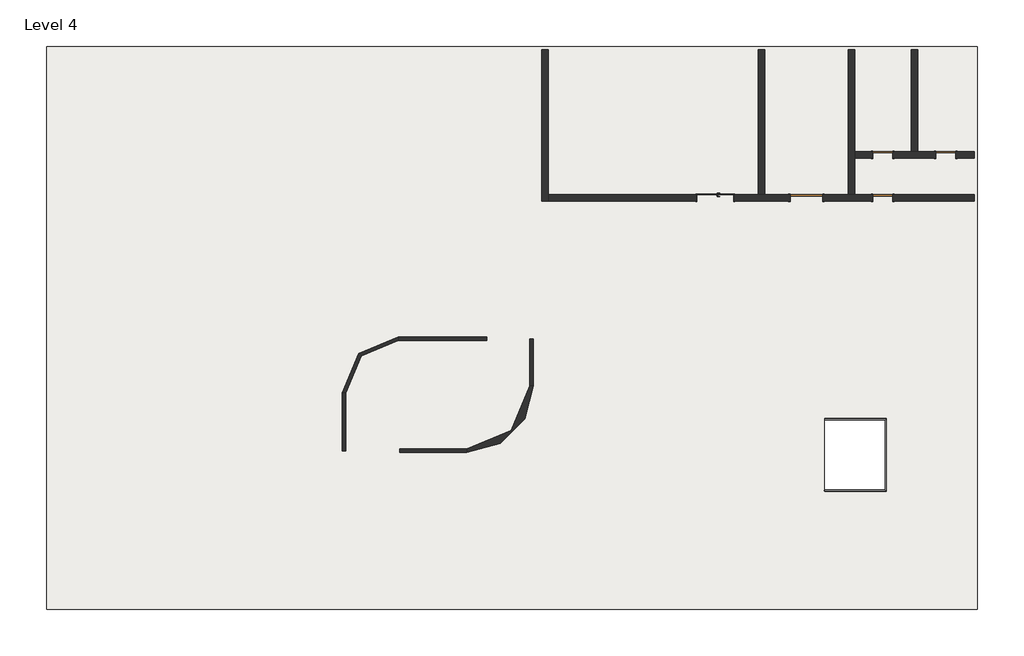
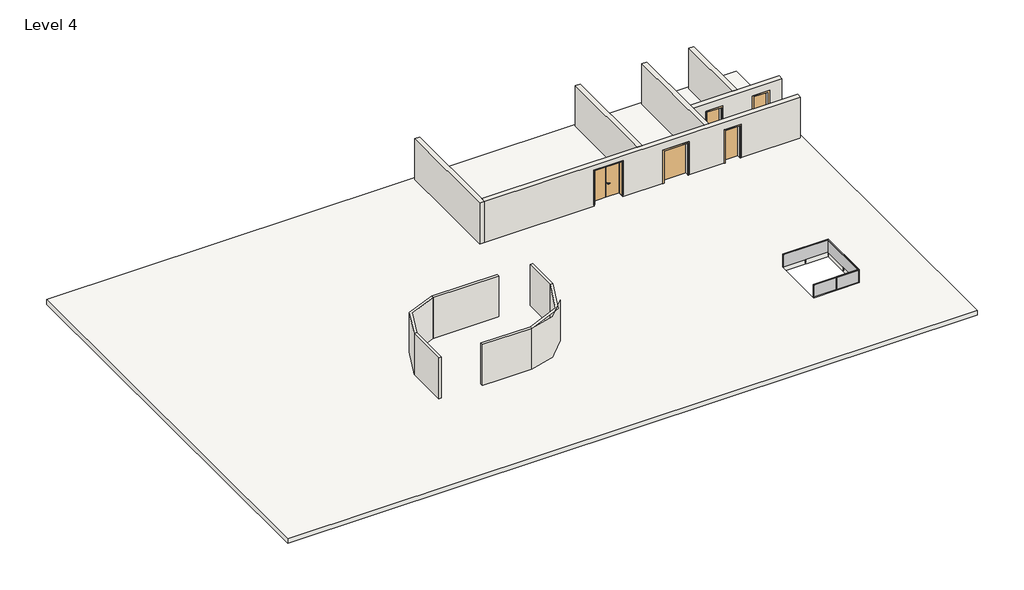
# One storey: 12 walls, 5 doors, 1 railing, 1 slab.
"""IFC4 building model written with IfcOpenShell, lengths in millimetres."""

import ifcopenshell
import ifcopenshell.guid

model = None  # the IFC model being written
_history = None  # IfcOwnerHistory: only IFC2X3 demands one
_inside = {}  # id of a spatial element -> (the spatial element, [elements in it])
_under = {}  # id of a project, library or spatial element -> (it, [spatial elements below it])
_declared = {}  # id of a project -> (the project, [libraries it declares])
_typed = {}  # id of a type object -> (the type object, [elements of that type])
_made_of = {}  # id of a material, layer set ... -> (it, [elements and type objects made of it])


def new_model(schema):
    """Start an empty IFC model of exactly this schema.

    Asked for "IFC4X3", IfcOpenShell would pick the latest addendum, in which some entities
    have other attributes; the version numbers below select the first issue.
    IFC2X3 requires an IfcOwnerHistory on every rooted entity: one is made here for all.
    """
    global model, _history
    if schema == "IFC4X3":
        model = ifcopenshell.file(schema_version=(4, 3, 0, 0))
    else:
        model = ifcopenshell.file(schema=schema)
    _inside.clear()
    _under.clear()
    _declared.clear()
    _typed.clear()
    _made_of.clear()
    _history = None
    if model.schema == "IFC2X3":
        org = make("IfcOrganization", Name="unknown")
        user = make(
            "IfcPersonAndOrganization",
            ThePerson=make("IfcPerson", FamilyName="unknown"),
            TheOrganization=org,
        )
        app = make(
            "IfcApplication",
            ApplicationDeveloper=org,
            Version="unknown",
            ApplicationFullName="unknown",
            ApplicationIdentifier="unknown",
        )
        _history = make(
            "IfcOwnerHistory",
            OwningUser=user,
            OwningApplication=app,
            ChangeAction="ADDED",
            CreationDate=0,
        )
    return model


def make(cls, **values):
    """One entity of the class cls with the attributes given. An attribute that is None is left unset."""
    return model.create_entity(
        cls, **{name: value for name, value in values.items() if value is not None}
    )


def rooted(cls, **values):
    """An entity with a GlobalId (a new one), such as an element, a storey or a relation."""
    return make(cls, GlobalId=ifcopenshell.guid.new(), OwnerHistory=_history, **values)


def si_unit(unit_type, name, prefix=None):
    """IfcSIUnit, for example si_unit("LENGTHUNIT", "METRE", prefix="MILLI")."""
    return make("IfcSIUnit", UnitType=unit_type, Prefix=prefix, Name=name)


def assignment(units):
    """IfcUnitAssignment: the units of a project."""
    return None if units is None else make("IfcUnitAssignment", Units=units)


def point(xyz):
    """IfcCartesianPoint."""
    return None if xyz is None else make("IfcCartesianPoint", Coordinates=xyz)


def direction(xyz):
    """IfcDirection."""
    return None if xyz is None else make("IfcDirection", DirectionRatios=xyz)


def frame(location, z_axis=None, x_axis=None):
    """IfcAxis2Placement3D, a coordinate frame: its origin and axes. An axis left out is left unset."""
    return make(
        "IfcAxis2Placement3D",
        Location=point(location),
        Axis=direction(z_axis),
        RefDirection=direction(x_axis),
    )


def frame_2d(location, x_axis=None):
    """IfcAxis2Placement2D, a coordinate frame in the plane: its origin and x axis."""
    return make(
        "IfcAxis2Placement2D", Location=point(location), RefDirection=direction(x_axis)
    )


def origin():
    """The frame at (0, 0, 0) with its axes left unset."""
    return frame((0.0, 0.0, 0.0))


def origin_with_axes():
    """The frame at (0, 0, 0) with the z axis (0, 0, 1) and the x axis (1, 0, 0) written out."""
    return frame((0.0, 0.0, 0.0), z_axis=(0.0, 0.0, 1.0), x_axis=(1.0, 0.0, 0.0))


def place(relative_to, where):
    """IfcLocalPlacement: puts the frame where relative to a parent placement (None: the world)."""
    return make(
        "IfcLocalPlacement", PlacementRelTo=relative_to, RelativePlacement=where
    )


def context(
    kind, dimensions, precision=None, world=None, true_north=None, identifier=None
):
    """IfcGeometricRepresentationContext, for example the 3D "Model" context."""
    return make(
        "IfcGeometricRepresentationContext",
        ContextIdentifier=identifier,
        ContextType=kind,
        CoordinateSpaceDimension=dimensions,
        Precision=precision,
        WorldCoordinateSystem=world,
        TrueNorth=true_north,
    )


def project(units=None, contexts=None):
    """IfcProject with its units and contexts."""
    return rooted(
        "IfcProject",
        Name="project",
        RepresentationContexts=contexts,
        UnitsInContext=assignment(units),
    )


def spatial(cls, under=None, at=None, **own):
    """A site, building, storey or space (cls), placed at a placement, below another one or the project."""
    s = rooted(cls, ObjectPlacement=at, **own)
    if under is not None:
        _under.setdefault(under.id(), (under, []))[1].append(s)
    return s


def polyline(points):
    """IfcPolyline through the points."""
    return make("IfcPolyline", Points=[point(p) for p in points])


def circle_curve(where, radius):
    """IfcCircle in the frame where."""
    return make("IfcCircle", Position=where, Radius=radius)


def ellipse_curve(where, semi_axis1, semi_axis2):
    """IfcEllipse in the frame where."""
    return make(
        "IfcEllipse", Position=where, SemiAxis1=semi_axis1, SemiAxis2=semi_axis2
    )


def trimmed(basis, trim1, trim2, sense, master):
    """IfcTrimmedCurve: the piece of a basis curve between two trims."""
    return make(
        "IfcTrimmedCurve",
        BasisCurve=basis,
        Trim1=trim1,
        Trim2=trim2,
        SenseAgreement=sense,
        MasterRepresentation=master,
    )


def segment(curve, same_sense, transition):
    """IfcCompositeCurveSegment."""
    return make(
        "IfcCompositeCurveSegment",
        Transition=transition,
        SameSense=same_sense,
        ParentCurve=curve,
    )


def composite_curve(segments, self_intersect=None):
    """IfcCompositeCurve: segments joined end to end."""
    return make("IfcCompositeCurve", Segments=segments, SelfIntersect=self_intersect)


def outline(outer, holes=None, kind="AREA"):
    """IfcArbitraryClosedProfileDef: a profile drawn as a closed curve; with holes, ...WithVoids."""
    if holes is None:
        return make("IfcArbitraryClosedProfileDef", ProfileType=kind, OuterCurve=outer)
    return make(
        "IfcArbitraryProfileDefWithVoids",
        ProfileType=kind,
        OuterCurve=outer,
        InnerCurves=holes,
    )


def extrude(swept, where, along, depth):
    """IfcExtrudedAreaSolid: the profile swept, set in the frame where, extruded along a direction by depth."""
    return make(
        "IfcExtrudedAreaSolid",
        SweptArea=swept,
        Position=where,
        ExtrudedDirection=direction(along),
        Depth=depth,
    )


def faces_of(points, faces, orient=None, outer=None):
    """IfcFace entities. A face is a list of loops; a loop is a list of indices into points, from 0.

    orient and outer hold one flag for each loop. By default every Orientation is true, the
    first loop of a face is its IfcFaceOuterBound and the others are IfcFaceBound.
    """
    made = []
    for i, loops in enumerate(faces):
        bounds = []
        for j, loop in enumerate(loops):
            is_outer = j == 0 if outer is None else outer[i][j]
            bounds.append(
                make(
                    "IfcFaceOuterBound" if is_outer else "IfcFaceBound",
                    Bound=make("IfcPolyLoop", Polygon=[points[k] for k in loop]),
                    Orientation=True if orient is None else orient[i][j],
                )
            )
        made.append(make("IfcFace", Bounds=bounds))
    return made


def faceted_brep(points, faces, orient=None, outer=None, voids=None):
    """IfcFacetedBrep: a solid bounded by flat faces; with voids (closed shells), ...WithVoids."""
    shared = [point(p) for p in points]
    hull = make("IfcClosedShell", CfsFaces=faces_of(shared, faces, orient, outer))
    if voids is None:
        return make("IfcFacetedBrep", Outer=hull)
    return make(
        "IfcFacetedBrepWithVoids",
        Outer=hull,
        Voids=[
            make(cls, CfsFaces=faces_of(shared, fs, o, b)) for cls, fs, o, b in voids
        ],
    )


def shape(context_of_items, identifier, shape_type, items):
    """IfcShapeRepresentation: the items that make up one representation, for example the "Body"."""
    return make(
        "IfcShapeRepresentation",
        ContextOfItems=context_of_items,
        RepresentationIdentifier=identifier,
        RepresentationType=shape_type,
        Items=items,
    )


def source(mapping_origin, context_of_items, identifier, shape_type, items):
    """IfcRepresentationMap: a shape defined once, which mapped items show again and again."""
    return make(
        "IfcRepresentationMap",
        MappingOrigin=mapping_origin,
        MappedRepresentation=shape(context_of_items, identifier, shape_type, items),
    )


def transform(
    local_origin,
    x_axis=None,
    y_axis=None,
    z_axis=None,
    scale=None,
    scale2=None,
    scale3=None,
    uniform=True,
):
    """IfcCartesianTransformationOperator3D, or its non-uniform kind. x_axis, y_axis, z_axis: its Axis1, 2, 3."""
    if uniform:
        return make(
            "IfcCartesianTransformationOperator3D",
            Axis1=direction(x_axis),
            Axis2=direction(y_axis),
            LocalOrigin=point(local_origin),
            Scale=scale,
            Axis3=direction(z_axis),
        )
    return make(
        "IfcCartesianTransformationOperator3DnonUniform",
        Axis1=direction(x_axis),
        Axis2=direction(y_axis),
        LocalOrigin=point(local_origin),
        Scale=scale,
        Axis3=direction(z_axis),
        Scale2=scale2,
        Scale3=scale3,
    )


def mapped(mapping_source, mapping_target):
    """IfcMappedItem: shows the shape of a source again, moved by a transform."""
    return make(
        "IfcMappedItem", MappingSource=mapping_source, MappingTarget=mapping_target
    )


def made_of(thing, what):
    """Note that an element or type object is made of a material, layer set ...; save() writes the relation."""
    if what is not None:
        _made_of.setdefault(what.id(), (what, []))[1].append(thing)
    return thing


def element(
    cls,
    number,
    at=None,
    inside=None,
    cuts=None,
    type_object=None,
    material=None,
    context=None,
    identifier="Body",
    shape_type=None,
    held_by="IfcProductDefinitionShape",
    body=None,
    shapes=None,
    **own,
):
    """One element of the class cls, such as IfcWall. Its Tag is "e" and its number.

    at: its placement. inside: the storey or other place that contains it. cuts: it is an
    opening in that element (IfcRelVoidsElement). A single representation is given by context,
    identifier, shape_type and body (its items); several are given by shapes. held_by: the class
    of the entity that holds the representations. save() writes the other relations.
    """
    e = rooted(cls, Tag="e%d" % number, ObjectPlacement=at, **own)
    if body is not None:
        shapes = [shape(context, identifier, shape_type, body)]
    if shapes is not None:
        e.Representation = make(held_by, Representations=shapes)
    if inside is not None:
        _inside.setdefault(inside.id(), (inside, []))[1].append(e)
    if cuts is not None:
        rooted(
            "IfcRelVoidsElement", RelatingBuildingElement=cuts, RelatedOpeningElement=e
        )
    if type_object is not None:
        _typed.setdefault(type_object.id(), (type_object, []))[1].append(e)
    return made_of(e, material)


def aggregate(whole, parts):
    """IfcRelAggregates: a whole, such as a stair, and the parts it consists of."""
    return rooted("IfcRelAggregates", RelatingObject=whole, RelatedObjects=parts)


def save(model, path):
    """Write the relations noted so far, then the file.

    IfcRelAggregates (storeys below a building ...), IfcRelContainedInSpatialStructure (elements
    in a storey), IfcRelDefinesByType, IfcRelAssociatesMaterial and IfcRelDeclares: one each for
    every whole, place, type object, material and project.
    """
    for whole, parts in _under.values():
        aggregate(whole, parts)
    for where, things in _inside.values():
        rooted(
            "IfcRelContainedInSpatialStructure",
            RelatedElements=things,
            RelatingStructure=where,
        )
    for kind, things in _typed.values():
        rooted("IfcRelDefinesByType", RelatedObjects=things, RelatingType=kind)
    for what, things in _made_of.values():
        rooted("IfcRelAssociatesMaterial", RelatedObjects=things, RelatingMaterial=what)
    for by, libraries in _declared.values():
        rooted("IfcRelDeclares", RelatingContext=by, RelatedDefinitions=libraries)
    model.write(path)


def plane_surface(at):
    """IfcPlane: the flat surface through the origin of the frame at, square to its z axis."""
    return make("IfcPlane", Position=at)


def cylinder_surface(at, radius):
    """IfcCylindricalSurface: all points at the distance radius from the z axis of the frame at."""
    return make("IfcCylindricalSurface", Position=at, Radius=radius)


def advanced_brep(points, edges, surfaces, faces):
    """IfcAdvancedBrep: a solid bounded by faces that lie on surfaces and meet in shared edges.

    An edge is (start, end): straight between two places in points (the first is 0);
    or (start, end, curve); or (start, end, curve, False) where it runs against its curve.
    A face is (place in surfaces, loops), or (place, loops, False) where it looks against
    its surface's normal. A loop lists edges by number (the first is 1), with a minus sign
    where the edge is run from its end to its start. The first loop is the outer one.
    """
    corners = [point(p) for p in points]
    vertices = [make("IfcVertexPoint", VertexGeometry=c) for c in corners]
    made = []
    for start, end, *more in edges:
        made.append(
            make(
                "IfcEdgeCurve",
                EdgeStart=vertices[start],
                EdgeEnd=vertices[end],
                EdgeGeometry=more[0] if more else make("IfcPolyline", Points=[corners[start], corners[end]]),
                SameSense=more[1] if len(more) > 1 else True,
            )
        )
    hull = []
    for where, loops, *sense in faces:
        bounds = []
        for j, loop in enumerate(loops):
            ring = [make("IfcOrientedEdge", EdgeElement=made[abs(k) - 1], Orientation=k > 0) for k in loop]
            bounds.append(
                make(
                    "IfcFaceOuterBound" if j == 0 else "IfcFaceBound",
                    Bound=make("IfcEdgeLoop", EdgeList=ring),
                    Orientation=True,
                )
            )
        hull.append(make("IfcAdvancedFace", Bounds=bounds, FaceSurface=surfaces[where], SameSense=sense[0] if sense else True))
    return make("IfcAdvancedBrep", Outer=make("IfcClosedShell", CfsFaces=hull))


def door_double_flush_variable_door_double_flush_variable_ac6c3b87(model_context):
    return source(origin(), model_context, "Body", "SolidModel", [
        advanced_brep(
        [(90.0, 139.4346141, 1000.0), (110.0, 139.4346141, 1000.0), (90.0, 69.4346141, 1000.0), (110.0, 89.4346141, 1000.0), (220.0, 69.4346141, 1000.0), (220.0, 89.4346141, 1000.0)],
        [
            (0, 1, circle_curve(frame((100.0, 139.4346141, 1000.0), z_axis=(0.0, 1.0, 0.0), x_axis=(1.0, 0.0, 0.0)), 10.0)),
            (1, 0, circle_curve(frame((100.0, 139.4346141, 1000.0), z_axis=(0.0, 1.0, 0.0), x_axis=(1.0, 0.0, 0.0)), 10.0)),
            (0, 2),
            (2, 3, ellipse_curve(frame((100.0, 79.4346141, 1000.0), z_axis=(-0.7071067811865385, 0.7071067811865565, 0.0), x_axis=(0.7071067811865563, 0.7071067811865386, 0.0)), 14.1421356, 10.0)),
            (3, 1),
            (3, 2, ellipse_curve(frame((100.0, 79.4346141, 1000.0), z_axis=(-0.7071067811865385, 0.7071067811865565, 0.0), x_axis=(0.7071067811865563, 0.7071067811865386, 0.0)), 14.1421356, 10.0)),
            (4, 5, circle_curve(frame((220.0, 79.4346141, 1000.0), z_axis=(1.0, 0.0, 0.0), x_axis=(0.0, 1.0, 0.0)), 10.0)),
            (5, 4, circle_curve(frame((220.0, 79.4346141, 1000.0), z_axis=(1.0, 0.0, 0.0), x_axis=(0.0, 1.0, 0.0)), 10.0)),
            (2, 4),
            (5, 3),
        ],
        [
            plane_surface(frame((100.0, 139.4346141, -287.7526403), z_axis=(0.0, 1.0, 0.0), x_axis=(0.0, 0.0, 1.0))),
            cylinder_surface(frame((100.0, 139.4346141, 1000.0), z_axis=(0.0, 1.0, 0.0), x_axis=(1.0, 0.0, 0.0)), 10.0),
            plane_surface(frame((220.0, 79.4346141, -287.7526403), z_axis=(1.0, 0.0, 0.0), x_axis=(0.0, 0.0, 1.0))),
            cylinder_surface(frame((100.0, 79.4346141, 1000.0), z_axis=(-1.0, 0.0, 0.0), x_axis=(0.0, 1.0, 0.0)), 10.0),
        ],
        [
            (0, [[1, 2]]),
            (1, [[-1, 3, 4, 5]]),
            (1, [[-2, -5, 6, -3]]),
            (2, [[7, 8]]),
            (3, [[-4, 9, -8, 10]]),
            (3, [[-6, -10, -7, -9]]),
        ],
    ),
        advanced_brep(
        [(110.0, 199.4346141, 1000.0), (90.0, 199.4346141, 1000.0), (110.0, 229.4346141, 1000.0), (90.0, 249.4346141, 1000.0), (220.0, 229.4346141, 1000.0), (220.0, 249.4346141, 1000.0)],
        [
            (0, 1, circle_curve(frame((100.0, 199.4346141, 1000.0), z_axis=(0.0, -1.0, 0.0), x_axis=(-1.0, 0.0, 0.0)), 10.0)),
            (1, 0, circle_curve(frame((100.0, 199.4346141, 1000.0), z_axis=(0.0, -1.0, 0.0), x_axis=(-1.0, 0.0, 0.0)), 10.0)),
            (0, 2),
            (2, 3, ellipse_curve(frame((100.0, 239.4346141, 1000.0), z_axis=(-0.7071067811865475, -0.7071067811865475, 0.0), x_axis=(0.7071067811865474, -0.7071067811865476, 0.0)), 14.1421356, 10.0)),
            (3, 1),
            (3, 2, ellipse_curve(frame((100.0, 239.4346141, 1000.0), z_axis=(-0.7071067811865475, -0.7071067811865475, 0.0), x_axis=(0.7071067811865474, -0.7071067811865476, 0.0)), 14.1421356, 10.0)),
            (4, 5, circle_curve(frame((220.0, 239.4346141, 1000.0), z_axis=(1.0, 0.0, 0.0), x_axis=(0.0, 1.0, 0.0)), 10.0)),
            (5, 4, circle_curve(frame((220.0, 239.4346141, 1000.0), z_axis=(1.0, 0.0, 0.0), x_axis=(0.0, 1.0, 0.0)), 10.0)),
            (2, 4),
            (5, 3),
        ],
        [
            plane_surface(frame((100.0, 199.4346141, -287.7526403), z_axis=(0.0, -1.0, 0.0), x_axis=(0.0, 0.0, 1.0))),
            cylinder_surface(frame((100.0, 199.4346141, 1000.0), z_axis=(0.0, -1.0, 0.0), x_axis=(-1.0, 0.0, 0.0)), 10.0),
            plane_surface(frame((220.0, 239.4346141, -287.7526403), z_axis=(1.0, 0.0, 0.0), x_axis=(0.0, 0.0, 1.0))),
            cylinder_surface(frame((100.0, 239.4346141, 1000.0), z_axis=(-1.0, 0.0, 0.0), x_axis=(0.0, 1.0, 0.0)), 10.0),
        ],
        [
            (0, [[1, 2]]),
            (1, [[-1, 3, 4, 5]]),
            (1, [[-2, -5, 6, -3]]),
            (2, [[7, 8]]),
            (3, [[-4, 9, -8, 10]]),
            (3, [[-6, -10, -7, -9]]),
        ],
    ),
        extrude(outline(composite_curve([segment(trimmed(circle_curve(frame_2d((1000.0, 100.0)), 20.0), [point((1000.0, 80.0))], [point((1000.0, 120.0))], False, "CARTESIAN"), True, "CONTINUOUS"), segment(trimmed(circle_curve(frame_2d((1000.0, 100.0)), 20.0), [point((1000.0, 120.0))], [point((1000.0, 80.0))], False, "CARTESIAN"), True, "CONTINUOUS")], self_intersect=False)), frame((0.0, 129.4346141, 0.0), z_axis=(0.0, 1.0, 0.0), x_axis=(0.0, 0.0, 1.0)), (0.0, 0.0, 1.0), 10.0),
        extrude(outline(composite_curve([segment(trimmed(circle_curve(frame_2d((1000.0, 100.0)), 20.0), [point((1000.0, 80.0))], [point((1000.0, 120.0))], False, "CARTESIAN"), True, "CONTINUOUS"), segment(trimmed(circle_curve(frame_2d((1000.0, 100.0)), 20.0), [point((1000.0, 120.0))], [point((1000.0, 80.0))], False, "CARTESIAN"), True, "CONTINUOUS")], self_intersect=False)), frame((0.0, 189.4346141, 0.0), z_axis=(0.0, 1.0, 0.0), x_axis=(0.0, 0.0, 1.0)), (0.0, 0.0, 1.0), 10.0),
        extrude(outline(polyline([(0.0, 164.4346141), (-871.25, 164.4346141), (-871.25, 189.4346141), (0.0, 189.4346141), (0.0, 164.4346141)])), frame((0.0, 0.0, 100.0), z_axis=(0.0, 0.0, 1.0), x_axis=(1.0, 0.0, 0.0)), (0.0, 0.0, 1.0), 2250.0),
        extrude(outline(polyline([(871.25, 164.4346141), (0.0, 164.4346141), (0.0, 189.4346141), (871.25, 189.4346141), (871.25, 164.4346141)])), frame((0.0, 0.0, 100.0), z_axis=(0.0, 0.0, 1.0), x_axis=(1.0, 0.0, 0.0)), (0.0, 0.0, 1.0), 2250.0),
        faceted_brep([(905.75, -150.5653859, 100.0), (856.25, -150.5653859, 100.0), (856.25, 164.4346141, 100.0), (871.25, 164.4346141, 100.0), (871.25, 189.4346141, 100.0), (905.75, 189.4346141, 100.0), (905.75, 164.4346141, 100.0), (900.75, 164.4346141, 100.0), (900.75, 184.4346141, 100.0), (876.25, 184.4346141, 100.0), (876.25, 159.4346141, 100.0), (861.25, 159.4346141, 100.0), (861.25, -145.5653859, 100.0), (900.75, -145.5653859, 100.0), (900.75, -135.5653859, 100.0), (905.75, -135.5653859, 100.0), (905.75, -150.5653859, 2384.5), (-905.75, -150.5653859, 2384.5), (-905.75, -150.5653859, 100.0), (-856.25, -150.5653859, 100.0), (-856.25, -150.5653859, 2335.0), (856.25, -150.5653859, 2335.0), (856.25, 164.4346141, 2335.0), (-856.25, 164.4346141, 2335.0), (-856.25, 164.4346141, 100.0), (-871.25, 164.4346141, 100.0), (-871.25, 164.4346141, 2350.0), (871.25, 164.4346141, 2350.0), (871.25, 189.4346141, 2350.0), (-871.25, 189.4346141, 2350.0), (-871.25, 189.4346141, 100.0), (-905.75, 189.4346141, 100.0), (-905.75, 189.4346141, 2384.5), (905.75, 189.4346141, 2384.5), (905.75, 164.4346141, 2384.5), (-905.75, 164.4346141, 2384.5), (-905.75, 164.4346141, 100.0), (-900.75, 164.4346141, 100.0), (-900.75, 164.4346141, 2379.5), (900.75, 164.4346141, 2379.5), (900.75, 184.4346141, 2379.5), (-900.75, 184.4346141, 2379.5), (-900.75, 184.4346141, 100.0), (-876.25, 184.4346141, 100.0), (-876.25, 184.4346141, 2355.0), (876.25, 184.4346141, 2355.0), (876.25, 159.4346141, 2355.0), (-876.25, 159.4346141, 2355.0), (-876.25, 159.4346141, 100.0), (-861.25, 159.4346141, 100.0), (-861.25, 159.4346141, 2340.0), (861.25, 159.4346141, 2340.0), (861.25, -145.5653859, 2340.0), (-861.25, -145.5653859, 2340.0), (-861.25, -145.5653859, 100.0), (-900.75, -145.5653859, 100.0), (-900.75, -145.5653859, 2379.5), (900.75, -145.5653859, 2379.5), (900.75, -135.5653859, 2379.5), (-900.75, -135.5653859, 2379.5), (-900.75, -135.5653859, 100.0), (-905.75, -135.5653859, 100.0), (-905.75, -135.5653859, 2384.5), (905.75, -135.5653859, 2384.5)], [[[0, 1, 2, 3, 4, 5, 6, 7, 8, 9, 10, 11, 12, 13, 14, 15]], [[1, 0, 16, 17, 18, 19, 20, 21]], [[2, 1, 21, 22]], [[3, 2, 22, 23, 24, 25, 26, 27]], [[4, 3, 27, 28]], [[5, 4, 28, 29, 30, 31, 32, 33]], [[6, 5, 33, 34]], [[7, 6, 34, 35, 36, 37, 38, 39]], [[8, 7, 39, 40]], [[9, 8, 40, 41, 42, 43, 44, 45]], [[10, 9, 45, 46]], [[11, 10, 46, 47, 48, 49, 50, 51]], [[12, 11, 51, 52]], [[13, 12, 52, 53, 54, 55, 56, 57]], [[14, 13, 57, 58]], [[15, 14, 58, 59, 60, 61, 62, 63]], [[0, 15, 63, 16]], [[17, 62, 61, 18]], [[18, 61, 60, 55, 54, 49, 48, 43, 42, 37, 36, 31, 30, 25, 24, 19]], [[23, 20, 19, 24]], [[29, 26, 25, 30]], [[35, 32, 31, 36]], [[41, 38, 37, 42]], [[47, 44, 43, 48]], [[53, 50, 49, 54]], [[59, 56, 55, 60]], [[22, 21, 20, 23]], [[28, 27, 26, 29]], [[34, 33, 32, 35]], [[40, 39, 38, 41]], [[46, 45, 44, 47]], [[52, 51, 50, 53]], [[58, 57, 56, 59]], [[16, 63, 62, 17]]]),
    ])


def m_single_flush_0915_x_2134mm_1c84716f(model_context):
    return source(origin(), model_context, "Body", "SweptSolid", [
        extrude(outline(polyline([(2210.0, -533.5), (0.0, -533.5), (0.0, -457.5), (2134.0, -457.5), (2134.0, 457.5), (0.0, 457.5), (0.0, 533.5), (2210.0, 533.5), (2210.0, -533.5)])), frame((0.0, -175.0, 0.0), z_axis=(0.0, 1.0, 0.0), x_axis=(0.0, 0.0, 1.0)), (0.0, 0.0, 1.0), 25.0),
        extrude(outline(polyline([(2210.0, 533.5), (2210.0, -533.5), (0.0, -533.5), (0.0, -457.5), (2134.0, -457.5), (2134.0, 457.5), (0.0, 457.5), (0.0, 533.5), (2210.0, 533.5)])), frame((0.0, 150.0, 0.0), z_axis=(0.0, 1.0, 0.0), x_axis=(0.0, 0.0, 1.0)), (0.0, 0.0, 1.0), 25.0),
        extrude(outline(polyline([(457.5, -99.0), (457.5, -150.0), (-457.5, -150.0), (-457.5, -99.0), (457.5, -99.0)])), origin_with_axes(), (0.0, 0.0, 1.0), 2134.0),
    ])


def m_single_flush_1500_x_2134mm_2_edebd810(model_context):
    return source(origin(), model_context, "Body", "SweptSolid", [
        extrude(outline(polyline([(2210.0, -826.0), (0.0, -826.0), (0.0, -750.0), (2134.0, -750.0), (2134.0, 750.0), (0.0, 750.0), (0.0, 826.0), (2210.0, 826.0), (2210.0, -826.0)])), frame((0.0, -175.0, 0.0), z_axis=(0.0, 1.0, 0.0), x_axis=(0.0, 0.0, 1.0)), (0.0, 0.0, 1.0), 25.0),
        extrude(outline(polyline([(2210.0, 826.0), (2210.0, -826.0), (0.0, -826.0), (0.0, -750.0), (2134.0, -750.0), (2134.0, 750.0), (0.0, 750.0), (0.0, 826.0), (2210.0, 826.0)])), frame((0.0, 150.0, 0.0), z_axis=(0.0, 1.0, 0.0), x_axis=(0.0, 0.0, 1.0)), (0.0, 0.0, 1.0), 25.0),
        extrude(outline(polyline([(750.0, -99.0), (750.0, -150.0), (-750.0, -150.0), (-750.0, -99.0), (750.0, -99.0)])), origin_with_axes(), (0.0, 0.0, 1.0), 2134.0),
    ])


def glas_mpk_6e7e974a(model_context):
    return source(origin(), model_context, "Body", "SolidModel", [
        faceted_brep([(29194.1667192, -1196.642277, 9843.2628643), (29194.1667192, -1246.642277, 9843.2628643), (29194.1667192, -1246.642277, 9856.7371357), (29194.1667192, -1196.642277, 9856.7371357), (32034.1667192, -1196.642277, 9843.2628643), (31984.1667192, -1246.642277, 9843.2628643), (31984.1667192, -1246.642277, 9856.7371357), (32034.1667192, -1196.642277, 9856.7371357), (32034.1667192, -4537.3716232, 9843.2628643), (31984.1667192, -4487.3716232, 9843.2628643), (31984.1667192, -4487.3716232, 9856.7371357), (32034.1667192, -4537.3716232, 9856.7371357), (29194.1667192, -4537.3716232, 9843.2628643), (29194.1667192, -4537.3716232, 9856.7371357), (29194.1667192, -4487.3716232, 9856.7371357), (29194.1667192, -4487.3716232, 9843.2628643)], [[[0, 1, 2, 3]], [[1, 0, 4, 5]], [[2, 1, 5, 6]], [[3, 2, 6, 7]], [[0, 3, 7, 4]], [[5, 4, 8, 9]], [[6, 5, 9, 10]], [[7, 6, 10, 11]], [[4, 7, 11, 8]], [[12, 13, 14, 15]], [[9, 8, 12, 15]], [[10, 9, 15, 14]], [[11, 10, 14, 13]], [[8, 11, 13, 12]]]),
        faceted_brep([(29194.1667192, -1236.642277, 9842.8769824), (29194.1667192, -1222.4501531, 9842.8769824), (29194.1667192, -1222.4501531, 9042.8769824), (29194.1667192, -1236.642277, 9042.8769824), (31994.1667192, -1236.642277, 9842.8769824), (32008.3588432, -1222.4501531, 9842.8769824), (32008.3588432, -1222.4501531, 9042.8769824), (31994.1667192, -1236.642277, 9042.8769824), (31994.1667192, -4497.3716232, 9842.8769824), (32008.3588432, -4511.5637472, 9842.8769824), (32008.3588432, -4511.5637472, 9042.8769824), (31994.1667192, -4497.3716232, 9042.8769824), (29194.1667192, -4497.3716232, 9842.8769824), (29194.1667192, -4497.3716232, 9042.8769824), (29194.1667192, -4511.5637472, 9042.8769824), (29194.1667192, -4511.5637472, 9842.8769824)], [[[0, 1, 2, 3]], [[1, 0, 4, 5]], [[2, 1, 5, 6]], [[3, 2, 6, 7]], [[0, 3, 7, 4]], [[5, 4, 8, 9]], [[6, 5, 9, 10]], [[7, 6, 10, 11]], [[4, 7, 11, 8]], [[12, 13, 14, 15]], [[9, 8, 12, 15]], [[10, 9, 15, 14]], [[11, 10, 14, 13]], [[8, 11, 13, 12]]]),
        extrude(outline(polyline([(30625.4167192, -4512.3716232), (30625.4167192, -4537.3716232), (30600.4167192, -4537.3716232), (30600.4167192, -4512.3716232), (30625.4167192, -4512.3716232)])), frame((0.0, 0.0, 8800.0), z_axis=(0.0, 0.0, 1.0), x_axis=(1.0, 0.0, 0.0)), (0.0, 0.0, 1.0), 1043.2628643),
        extrude(outline(polyline([(32009.1667192, -2854.5069501), (32034.1667192, -2854.5069501), (32034.1667192, -2879.5069501), (32009.1667192, -2879.5069501), (32009.1667192, -2854.5069501)])), frame((0.0, 0.0, 8800.0), z_axis=(0.0, 0.0, 1.0), x_axis=(1.0, 0.0, 0.0)), (0.0, 0.0, 1.0), 1043.2628643),
        extrude(outline(polyline([(30600.4167192, -1221.642277), (30600.4167192, -1196.642277), (30625.4167192, -1196.642277), (30625.4167192, -1221.642277), (30600.4167192, -1221.642277)])), frame((0.0, 0.0, 8800.0), z_axis=(0.0, 0.0, 1.0), x_axis=(1.0, 0.0, 0.0)), (0.0, 0.0, 1.0), 1043.2628643),
        extrude(outline(polyline([(32009.1667192, -4522.3716232), (32034.1667192, -4522.3716232), (32034.1667192, -4547.3716232), (32009.1667192, -4547.3716232), (32009.1667192, -4522.3716232)])), frame((0.0, 0.0, 8800.0), z_axis=(0.0, 0.0, 1.0), x_axis=(1.0, 0.0, 0.0)), (0.0, 0.0, 1.0), 1043.2628643),
        extrude(outline(polyline([(32019.1667192, -1221.642277), (32019.1667192, -1196.642277), (32044.1667192, -1196.642277), (32044.1667192, -1221.642277), (32019.1667192, -1221.642277)])), frame((0.0, 0.0, 8800.0), z_axis=(0.0, 0.0, 1.0), x_axis=(1.0, 0.0, 0.0)), (0.0, 0.0, 1.0), 1043.2628643),
        extrude(outline(polyline([(29206.6667192, -4512.3716232), (29206.6667192, -4537.3716232), (29181.6667192, -4537.3716232), (29181.6667192, -4512.3716232), (29206.6667192, -4512.3716232)])), frame((0.0, 0.0, 8800.0), z_axis=(0.0, 0.0, 1.0), x_axis=(1.0, 0.0, 0.0)), (0.0, 0.0, 1.0), 1043.2628643),
        extrude(outline(polyline([(29194.1667192, -1221.642277), (29194.1667192, -1196.642277), (29219.1667192, -1196.642277), (29219.1667192, -1221.642277), (29194.1667192, -1221.642277)])), frame((0.0, 0.0, 8800.0), z_axis=(0.0, 0.0, 1.0), x_axis=(1.0, 0.0, 0.0)), (0.0, 0.0, 1.0), 1043.2628643),
    ])


model = new_model("IFC4")

# Units and contexts
model_context = context("Model", 3, world=origin())
ifc_project = project(units=[si_unit("LENGTHUNIT", "METRE", prefix="MILLI")], contexts=[model_context])

# Site, building, storey
site = spatial("IfcSite", under=ifc_project)
building = spatial("IfcBuilding", under=site)
storey = spatial("IfcBuildingStorey", under=building, Name="Level 4", Elevation=9000.0)

# Doors
placement = place(None, origin())
door_double_flush_variable_door_double_flush_variable_shape = door_double_flush_variable_door_double_flush_variable_ac6c3b87(model_context)
element("IfcDoor", 1, ObjectType="Door Double Flush - Variable : Door Double Flush - Variable", at=placement, inside=storey, context=model_context, shape_type="MappedRepresentation", body=[
    mapped(door_double_flush_variable_door_double_flush_variable_shape, transform((24136.7471367, 8984.3231089, 9000.0), x_axis=(1.0, 0.0, 0.0), y_axis=(0.0, 1.0, 0.0), z_axis=(0.0, 0.0, 1.0))),
])
m_single_flush_0915_x_2134mm_shape = m_single_flush_0915_x_2134mm_1c84716f(model_context)
element("IfcDoor", 2, ObjectType="M_Single-Flush : 0915 x 2134mm", at=placement, inside=storey, context=model_context, shape_type="MappedRepresentation", body=[
    mapped(m_single_flush_0915_x_2134mm_shape, transform((34787.1221367, 10998.757723, 9000.0), x_axis=(-1.0, 0.0, 0.0), y_axis=(0.0, -1.0, 0.0), z_axis=(0.0, 0.0, 1.0))),
])
element("IfcDoor", 3, ObjectType="M_Single-Flush : 0915 x 2134mm", at=placement, inside=storey, context=model_context, shape_type="MappedRepresentation", body=[
    mapped(m_single_flush_0915_x_2134mm_shape, transform((31874.3721367, 10998.757723, 9000.0), x_axis=(-1.0, 0.0, 0.0), y_axis=(0.0, -1.0, 0.0), z_axis=(0.0, 0.0, 1.0))),
])
element("IfcDoor", 4, ObjectType="M_Single-Flush : 0915 x 2134mm", at=placement, inside=storey, context=model_context, shape_type="MappedRepresentation", body=[
    mapped(m_single_flush_0915_x_2134mm_shape, transform((31874.3721367, 8998.757723, 9000.0), x_axis=(-1.0, 0.0, 0.0), y_axis=(0.0, -1.0, 0.0), z_axis=(0.0, 0.0, 1.0))),
])
m_single_flush_1500_x_2134mm_2_shape = m_single_flush_1500_x_2134mm_2_edebd810(model_context)
element("IfcDoor", 5, ObjectType="M_Single-Flush : 1500 x 2134mm 2", at=placement, inside=storey, context=model_context, shape_type="MappedRepresentation", body=[
    mapped(m_single_flush_1500_x_2134mm_2_shape, transform((28342.9971367, 8998.757723, 9000.0), x_axis=(-1.0, 0.0, 0.0), y_axis=(0.0, -1.0, 0.0), z_axis=(0.0, 0.0, 1.0))),
])

# Railing
glas_mpk_shape = glas_mpk_6e7e974a(model_context)
element("IfcRailing", 6, ObjectType="Glas - MPK", at=placement, inside=storey, context=model_context, shape_type="MappedRepresentation", body=[
    mapped(glas_mpk_shape, transform((0.0, 0.0, 0.0), x_axis=(1.0, 0.0, 0.0), y_axis=(0.0, 1.0, 0.0), z_axis=(0.0, 0.0, 1.0))),
])

# Slab
element("IfcSlab", 7, ObjectType="Generic 300mm", at=placement, inside=storey, context=model_context, shape_type="SweptSolid", body=[
    extrude(outline(polyline([(-6732.0028633, 15998.757723), (36243.4971367, 15998.757723), (36243.4971367, -10001.242277), (-6732.0028633, -10001.242277), (-6732.0028633, 15998.757723)]), holes=[polyline([(32044.1667192, -1186.642277), (29194.1667192, -1186.642277), (29194.1667192, -4547.3716232), (32044.1667192, -4547.3716232), (32044.1667192, -1186.642277)])]), frame((0.0, 0.0, 8700.0), z_axis=(0.0, 0.0, 1.0), x_axis=(1.0, 0.0, 0.0)), (0.0, 0.0, 1.0), 300.0),
])

# Walls
element("IfcWall", 8, ObjectType="Generic - 300mm", at=placement, inside=storey, context=model_context, shape_type="Brep", body=[
    faceted_brep([(16117.9971367, 15848.757723, 9000.0), (16117.9971367, 8848.757723, 9000.0), (16117.9971367, 8848.757723, 11700.0), (16117.9971367, 15848.757723, 11700.0), (16417.9971367, 15848.757723, 9000.0), (16417.9971367, 15848.757723, 11700.0), (16417.9971367, 9148.757723, 11700.0), (16417.9971367, 8848.757723, 11700.0), (16417.9971367, 8848.757723, 9000.0), (16417.9971367, 9148.757723, 9000.0)], [[[0, 1, 2, 3]], [[4, 5, 6, 7, 8, 9]], [[1, 0, 4, 9, 8]], [[3, 2, 7, 6, 5]], [[2, 1, 8, 7]], [[0, 3, 5, 4]]]),
])
element("IfcWall", 9, ObjectType="Generic - 300mm", at=placement, inside=storey, context=model_context, shape_type="SweptSolid", body=[
    extrude(outline(polyline([(26117.9971367, 9148.757723), (26117.9971367, 15848.757723), (26417.9971367, 15848.757723), (26417.9971367, 9148.757723), (26117.9971367, 9148.757723)])), frame((0.0, 0.0, 9000.0), z_axis=(0.0, 0.0, 1.0), x_axis=(1.0, 0.0, 0.0)), (0.0, 0.0, 1.0), 2700.0),
])
element("IfcWall", 10, ObjectType="Generic - 300mm", at=placement, inside=storey, context=model_context, shape_type="Brep", body=[
    faceted_brep([(30267.9971367, 15848.757723, 9000.0), (30267.9971367, 9148.757723, 9000.0), (30267.9971367, 9148.757723, 11700.0), (30267.9971367, 15848.757723, 11700.0), (30567.9971367, 15848.757723, 9000.0), (30567.9971367, 15848.757723, 11700.0), (30567.9971367, 11148.757723, 11700.0), (30567.9971367, 10848.757723, 11700.0), (30567.9971367, 9148.757723, 11700.0), (30567.9971367, 9148.757723, 9000.0), (30567.9971367, 10848.757723, 9000.0), (30567.9971367, 11148.757723, 9000.0)], [[[0, 1, 2, 3]], [[4, 5, 6, 7, 8, 9, 10, 11]], [[1, 0, 4, 11, 10, 9]], [[3, 2, 8, 7, 6, 5]], [[2, 1, 9, 8]], [[0, 3, 5, 4]]]),
])
element("IfcWall", 11, ObjectType="Generic - 300mm", at=placement, inside=storey, context=model_context, shape_type="SweptSolid", body=[
    extrude(outline(polyline([(33180.7471367, 11148.757723), (33180.7471367, 15848.757723), (33480.7471367, 15848.757723), (33480.7471367, 11148.757723), (33180.7471367, 11148.757723)])), frame((0.0, 0.0, 9000.0), z_axis=(0.0, 0.0, 1.0), x_axis=(1.0, 0.0, 0.0)), (0.0, 0.0, 1.0), 2700.0),
])
element("IfcWall", 12, ObjectType="Generic - 300mm", at=placement, inside=storey, context=model_context, shape_type="Brep", body=[
    faceted_brep([(16417.9971367, 9148.757723, 11700.0), (26117.9971367, 9148.757723, 11700.0), (26417.9971367, 9148.757723, 11700.0), (30267.9971367, 9148.757723, 11700.0), (30567.9971367, 9148.757723, 11700.0), (36093.4971367, 9148.757723, 11700.0), (36093.4971367, 9148.757723, 9000.0), (32331.8721367, 9148.757723, 9000.0), (32331.8721367, 9148.757723, 11134.0), (31416.8721367, 9148.757723, 11134.0), (31416.8721367, 9148.757723, 9000.0), (30567.9971367, 9148.757723, 9000.0), (30267.9971367, 9148.757723, 9000.0), (29092.9971367, 9148.757723, 9000.0), (29092.9971367, 9148.757723, 11134.0), (27592.9971367, 9148.757723, 11134.0), (27592.9971367, 9148.757723, 9000.0), (26417.9971367, 9148.757723, 9000.0), (26117.9971367, 9148.757723, 9000.0), (25017.9971367, 9148.757723, 9000.0), (25017.9971367, 9148.757723, 11360.0), (23255.4971367, 9148.757723, 11360.0), (23255.4971367, 9148.757723, 9000.0), (16417.9971367, 9148.757723, 9000.0), (36093.4971367, 8848.757723, 11700.0), (16417.9971367, 8848.757723, 11700.0), (16417.9971367, 8848.757723, 9000.0), (23255.4971367, 8848.757723, 9000.0), (23255.4971367, 8848.757723, 11360.0), (25017.9971367, 8848.757723, 11360.0), (25017.9971367, 8848.757723, 9000.0), (27592.9971367, 8848.757723, 9000.0), (27592.9971367, 8848.757723, 11134.0), (29092.9971367, 8848.757723, 11134.0), (29092.9971367, 8848.757723, 9000.0), (31416.8721367, 8848.757723, 9000.0), (31416.8721367, 8848.757723, 11134.0), (32331.8721367, 8848.757723, 11134.0), (32331.8721367, 8848.757723, 9000.0), (36093.4971367, 8848.757723, 9000.0)], [[[0, 1, 2, 3, 4, 5, 6, 7, 8, 9, 10, 11, 12, 13, 14, 15, 16, 17, 18, 19, 20, 21, 22, 23]], [[24, 25, 26, 27, 28, 29, 30, 31, 32, 33, 34, 35, 36, 37, 38, 39]], [[26, 23, 22, 27]], [[10, 35, 34, 13, 12, 11]], [[38, 7, 6, 39]], [[16, 31, 30, 19, 18, 17]], [[5, 4, 3, 2, 1, 0, 25, 24]], [[0, 23, 26, 25]], [[36, 35, 10, 9]], [[37, 36, 9, 8]], [[38, 37, 8, 7]], [[32, 31, 16, 15]], [[33, 32, 15, 14]], [[34, 33, 14, 13]], [[29, 20, 19, 30]], [[20, 29, 28, 21]], [[21, 28, 27, 22]], [[6, 5, 24, 39]]]),
])
element("IfcWall", 13, ObjectType="Generic - 300mm", at=placement, inside=storey, context=model_context, shape_type="Brep", body=[
    faceted_brep([(31416.8721367, 11148.757723, 11134.0), (31416.8721367, 11148.757723, 9000.0), (30567.9971367, 11148.757723, 9000.0), (30567.9971367, 11148.757723, 11700.0), (33180.7471367, 11148.757723, 11700.0), (33480.7471367, 11148.757723, 11700.0), (36093.4971367, 11148.757723, 11700.0), (36093.4971367, 11148.757723, 9000.0), (35244.6221367, 11148.757723, 9000.0), (35244.6221367, 11148.757723, 11134.0), (34329.6221367, 11148.757723, 11134.0), (34329.6221367, 11148.757723, 9000.0), (33480.7471367, 11148.757723, 9000.0), (33180.7471367, 11148.757723, 9000.0), (32331.8721367, 11148.757723, 9000.0), (32331.8721367, 11148.757723, 11134.0), (30567.9971367, 10848.757723, 9000.0), (31416.8721367, 10848.757723, 9000.0), (31416.8721367, 10848.757723, 11134.0), (32331.8721367, 10848.757723, 11134.0), (32331.8721367, 10848.757723, 9000.0), (34329.6221367, 10848.757723, 9000.0), (34329.6221367, 10848.757723, 11134.0), (35244.6221367, 10848.757723, 11134.0), (35244.6221367, 10848.757723, 9000.0), (36093.4971367, 10848.757723, 9000.0), (36093.4971367, 10848.757723, 11700.0), (30567.9971367, 10848.757723, 11700.0)], [[[0, 1, 2, 3, 4, 5, 6, 7, 8, 9, 10, 11, 12, 13, 14, 15]], [[16, 17, 18, 19, 20, 21, 22, 23, 24, 25, 26, 27]], [[8, 7, 25, 24]], [[2, 1, 17, 16]], [[14, 13, 12, 11, 21, 20]], [[6, 5, 4, 3, 27, 26]], [[3, 2, 16, 27]], [[22, 21, 11, 10]], [[23, 22, 10, 9]], [[24, 23, 9, 8]], [[18, 17, 1, 0]], [[19, 18, 0, 15]], [[20, 19, 15, 14]], [[7, 6, 26, 25]]]),
])
element("IfcWall", 14, ObjectType="Interior - Blockwork 140", at=placement, inside=storey, context=model_context, shape_type="SweptSolid", body=[
    extrude(outline(polyline([(13583.5160614, 2407.0363043), (9501.5160614, 2407.0363043), (9501.5160614, 2571.0363043), (13583.5160614, 2571.0363043), (13583.5160614, 2407.0363043)])), frame((0.0, 0.0, 9000.0), z_axis=(0.0, 0.0, 1.0), x_axis=(1.0, 0.0, 0.0)), (0.0, 0.0, 1.0), 2700.0),
])
element("IfcWall", 15, ObjectType="Interior - Blockwork 140", at=placement, inside=storey, context=model_context, shape_type="SweptSolid", body=[
    extrude(outline(polyline([(7083.5160614, -10.9636957), (7083.5160614, -2674.9636957), (6919.5160614, -2674.9636957), (6919.5160614, -10.9636957), (7083.5160614, -10.9636957)])), frame((0.0, 0.0, 9000.0), z_axis=(0.0, 0.0, 1.0), x_axis=(1.0, 0.0, 0.0)), (0.0, 0.0, 1.0), 2700.0),
])
element("IfcWall", 16, ObjectType="Interior - Blockwork 140", at=placement, inside=storey, context=model_context, shape_type="SweptSolid", body=[
    extrude(outline(polyline([(9583.5160614, -2592.9636957), (12665.5160614, -2592.9636957), (12665.5160614, -2756.9636957), (9583.5160614, -2756.9636957), (9583.5160614, -2592.9636957)])), frame((0.0, 0.0, 9000.0), z_axis=(0.0, 0.0, 1.0), x_axis=(1.0, 0.0, 0.0)), (0.0, 0.0, 1.0), 2700.0),
])
element("IfcWall", 17, ObjectType="Interior - Blockwork 140", at=placement, inside=storey, context=model_context, shape_type="SweptSolid", body=[
    extrude(outline(polyline([(15583.5160614, 325.0363043), (15583.5160614, 2489.0363043), (15747.5160614, 2489.0363043), (15747.5160614, 325.0363043), (15583.5160614, 325.0363043)])), frame((0.0, 0.0, 9000.0), z_axis=(0.0, 0.0, 1.0), x_axis=(1.0, 0.0, 0.0)), (0.0, 0.0, 1.0), 2700.0),
])
element("IfcWall", 18, ObjectType="Interior - Blockwork 140", at=placement, inside=storey, context=model_context, shape_type="SweptSolid", body=[
    extrude(outline(composite_curve([segment(polyline([(7083.5160614, -10.9636957), (6919.5160614, -10.9636957)]), True, "CONTINUOUS"), segment(trimmed(circle_curve(frame_2d((9501.5160614, -10.9636957)), 2582.0), [point((6919.5160614, -10.9636957))], [point((9501.5160614, 2571.0363043))], False, "CARTESIAN"), True, "CONTINUOUS"), segment(polyline([(9501.5160614, 2571.0363043), (9501.5160614, 2407.0363043)]), True, "CONTINUOUS"), segment(trimmed(circle_curve(frame_2d((9501.5160614, -10.9636957)), 2418.0), [point((9501.5160614, 2407.0363043))], [point((7083.5160614, -10.9636957))], True, "CARTESIAN"), True, "CONTINUOUS")], self_intersect=False)), frame((0.0, 0.0, 9000.0), z_axis=(0.0, 0.0, 1.0), x_axis=(1.0, 0.0, 0.0)), (0.0, 0.0, 1.0), 2700.0),
])
element("IfcWall", 19, ObjectType="Interior - Blockwork 140", at=placement, inside=storey, context=model_context, shape_type="SweptSolid", body=[
    extrude(outline(composite_curve([segment(polyline([(15583.5160614, 325.0363043), (15747.5160614, 325.0363043)]), True, "CONTINUOUS"), segment(trimmed(circle_curve(frame_2d((12665.5160614, 325.0363043)), 3082.0), [point((15747.5160614, 325.0363043))], [point((12665.5160614, -2756.9636957))], False, "CARTESIAN"), True, "CONTINUOUS"), segment(polyline([(12665.5160614, -2756.9636957), (12665.5160614, -2592.9636957)]), True, "CONTINUOUS"), segment(trimmed(circle_curve(frame_2d((12665.5160614, 325.0363043)), 2918.0), [point((12665.5160614, -2592.9636957))], [point((15583.5160614, 325.0363043))], True, "CARTESIAN"), True, "CONTINUOUS")], self_intersect=False)), frame((0.0, 0.0, 9000.0), z_axis=(0.0, 0.0, 1.0), x_axis=(1.0, 0.0, 0.0)), (0.0, 0.0, 1.0), 2700.0),
])

save(model, "model.ifc")

# Revit data of these elements
# Type "Door Double Flush - Variable : Door Double Flush - Variable"
#   Type Mark = "33"
#   Operation = "DoubleDoorSingleSwing"
#   Keynote = "16.03"
#   Rough Width [instance default] = 2.010 m
#   Rough Height [instance default] = 2.360 m
#   Doorhandle Height = 0.900 m
#   Height [instance default] = 2.260 m
#   Sill Height [instance default] = 0.100 m
#   Width [instance default] = 2.010 m
#   Visibility [instance default] = yes
#   Doorhandle choose [instance default] = element 138974
#   Doorhandle [instance default] = Metal _ Chrome
#   Door [instance default] = Door - Wood
#   Frame [instance default] = Door - Wood
#   Function = (empty or 0)
#   Wall Closure = (empty or 0)
#   Assembly Code = ""
# Type "M_Single-Flush : 0915 x 2134mm"
#   Type Mark = "20"
#   Thickness = 0.051 m
#   Height = 2.134 m
#   Trim Projection Ext = 0.025 m
#   Trim Projection Int = 0.025 m
#   Trim Width = 0.076 m
#   Width = 0.915 m
#   Door Material = Door - Panel
#   Frame Material = Door - Frame
#   Function = (empty or 0)
#   Wall Closure = (empty or 0)
# Type "M_Single-Flush : 1500 x 2134mm 2"
#   Type Mark = "34"
#   Thickness = 0.051 m
#   Height = 2.134 m
#   Trim Projection Ext = 0.025 m
#   Trim Projection Int = 0.025 m
#   Trim Width = 0.076 m
#   Width = 1.500 m
#   Door Material = Door - Panel
#   Frame Material = Door - Frame
#   Function = (empty or 0)
#   Wall Closure = (empty or 0)
# Type "Glas - MPK"
#   built-in parameter 1008619 = -0.0410105 (stored number, unit not read)
#   built-in parameter 1008612 = 0.019685 (stored number, unit not read)
#   built-in parameter 1008611 = 0.0984252 (stored number, unit not read)
#   built-in parameter 1008609 = 6.56168 (stored number, unit not read)
#   built-in parameter 1008604 = 0.19685 (stored number, unit not read)
#   built-in parameter 1008603 = 0.164042 (stored number, unit not read)
#   Railing Height = 0.865 m
#   built-in parameter 1008630 = 2
#   built-in parameter 1008610 = 1
#   built-in parameter 1008605 = 1
# Type "Generic 300mm"
#   Function = 0
#   Layers, outside or top first: 0.300 m no material (function 1)
# Type "Generic - 300mm"
#   Layers, outside or top first: 0.300 m no material (function 1)
# Type "Interior - Blockwork 140"
#   Layers, outside or top first: 0.012 m "Plasterboard" (function 5); 0.140 m "Masonry - Concrete Block" (function 1); 0.012 m "Plasterboard" (function 5)
# Element 1 (IfcDoor, "Door Double Flush - Variable : Door Double Flush - Variable")
#   Width = 1.7625 m
#   Sill Height = 0.100 m
#   Rough Width = 1.7625 m
#   Rough Height = 2.360 m
#   Height = 2.260 m
#   Visibility = yes
#   Frame = Door - Wood
#   Doorhandle choose = element 138974
#   Doorhandle = Metal _ Chrome
#   Door = Door - Wood
#   Phase Created = New Construction
#   Materials on its faces: "Door - Wood", "Metal _ Chrome"
# Elements 2, 3, 4 (IfcDoor, "M_Single-Flush : 0915 x 2134mm")
#   Phase Created = New Construction
#   Materials on its faces: "Door - Frame", "Door - Panel"
# Element 5 (IfcDoor, "M_Single-Flush : 1500 x 2134mm 2")
#   Phase Created = New Construction
#   Materials on its faces: "Door - Frame", "Door - Panel"
# Element 6 (IfcRailing, "Glas - MPK")
#   Phase Created = New Construction
#   Materials on its faces: "Metal - Aluminum", "Window - Glass"
# Element 7 (IfcSlab, "Generic 300mm")
#   built-in parameter 1001955 = 3.14159 (stored number, unit not read)
#   Height Offset From Level = 0.000 m
#   Phase Created = New Construction
#   Materials on its faces: "Default Floor"
# Elements 8, 9, 10, 11, 12, 13 (IfcWall, "Generic - 300mm")
#   Top Offset = -0.300 m
#   Base Offset = 0.000 m
#   wall height = 2.700 m
#   Phase Created = New Construction
#   Base Constraint = Level 4
#   Top Constraint = Level 5
#   Materials on its faces: "Default Wall"
# Elements 14, 15, 16, 17 (IfcWall, "Interior - Blockwork 140")
#   Top Offset = -0.300 m
#   Base Offset = 0.000 m
#   wall height = 2.700 m
#   Phase Created = New Construction
#   Base Constraint = Level 4
#   Top Constraint = Level 5
#   Materials on its faces: "Default Wall", "Plasterboard"
# Elements 18, 19 (IfcWall, "Interior - Blockwork 140")
#   Top Offset = -0.300 m
#   Base Offset = 0.000 m
#   Unconnected Height = 4.000 m
#   wall height = 2.700 m
#   Phase Created = New Construction
#   Materials on its faces: "Default Wall", "Plasterboard"
# Materials
#   "Metal _ Chrome": class "Metall", colour RGB 247 247 247, transparency 0
#   "Door - Wood": class "Unassigned", colour RGB 114 94 79, transparency 0
#   "Door - Panel": class "Wood", colour RGB 210 159 95, transparency 0
#   "Door - Frame": class "Miscellaneous", colour RGB 118 70 51, transparency 0
#   "Plasterboard": class "Drywall", colour RGB 249 249 249, transparency 0, Description = "Interior finish"
#   "Masonry - Concrete Block": class "Concrete", colour RGB 181 181 181, transparency 0
#   "Metal - Aluminum": class "Unassigned", colour RGB 247 247 247, transparency 0, Comments = "Rendering appearance not upgraded "
#   "Window - Glass": class "Glas", colour RGB 128 128 255, transparency 0.75
#   "Default Floor": class "Miscellaneous", colour RGB 127 127 127, transparency 0
#   "Default Wall": class "Miscellaneous", colour RGB 128 128 128, transparency 0
